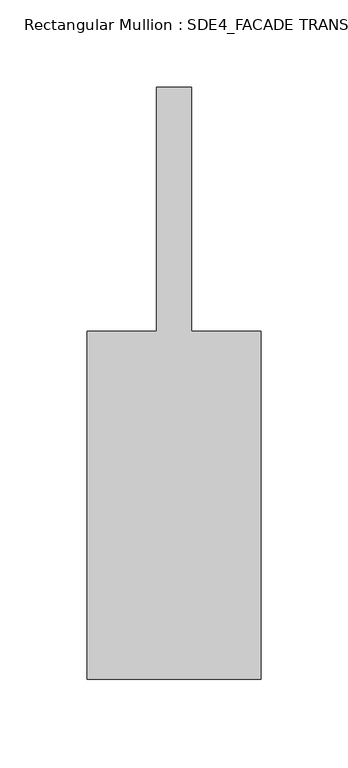
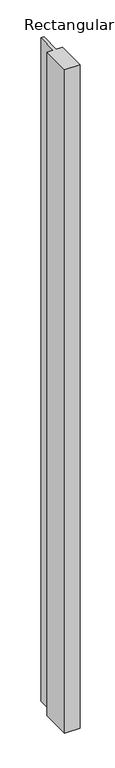
"""IFC4 building model written with IfcOpenShell, lengths in millimetres: member geometry, Rectangular Mullion : SDE4_FACADE TRANSOM TYPE 1."""

from ifc_helpers import new_model, si_unit, frame, origin, place, context, project, spatial, polyline, outline, extrude, source, transform, mapped, element, save


def rectangular_mullion_sde4_facade_transom_type_1_2f9a268f(model_context):
    return source(origin(), model_context, "Body", "SweptSolid", [
        extrude(outline(polyline([(50.0, -132.5), (-50.0, -132.5), (-50.0, 67.5), (-10.0, 67.5), (-10.0, 207.5), (10.0, 207.5), (10.0, 67.5), (50.0, 67.5), (50.0, -132.5)])), frame((0.0, 0.0, -4578.0), z_axis=(0.0, 0.0, 1.0), x_axis=(1.0, 0.0, 0.0)), (0.0, 0.0, 1.0), 4578.0),
    ])


if __name__ == "__main__":
    model = new_model("IFC4")
    model_context = context("Model", 3, world=origin())
    ifc_project = project(units=[si_unit("LENGTHUNIT", "METRE", prefix="MILLI")], contexts=[model_context])
    site = spatial("IfcSite", under=ifc_project)
    building = spatial("IfcBuilding", under=site)
    placement = place(None, origin())
    rectangular_mullion_sde4_facade_transom_type_1_shape = rectangular_mullion_sde4_facade_transom_type_1_2f9a268f(model_context)
    element("IfcMember", 1, ObjectType="Rectangular Mullion : SDE4_FACADE TRANSOM TYPE 1", at=placement, inside=building, context=model_context, shape_type="MappedRepresentation", body=[
        mapped(rectangular_mullion_sde4_facade_transom_type_1_shape, transform((0.0, 0.0, 0.0), x_axis=(1.0, 0.0, 0.0), y_axis=(0.0, 1.0, 0.0), z_axis=(0.0, 0.0, 1.0))),
    ])
    save(model, "model.ifc")

# Revit data of these elements
# Type "Rectangular Mullion : SDE4_FACADE TRANSOM TYPE 1"
#   built-in parameter 1007322 = 1.11549 (stored number, unit not read)
#   built-in parameter 1007321 = 0.164042 (stored number, unit not read)
#   built-in parameter 1007320 = 0.164042 (stored number, unit not read)
